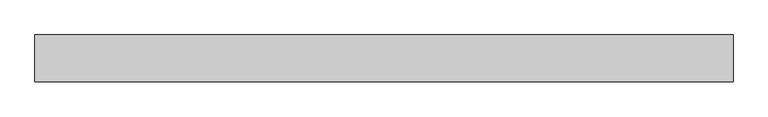
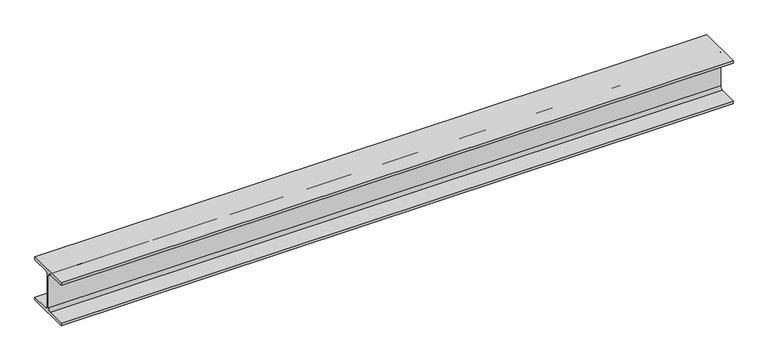
"""IFC4 building model written with IfcOpenShell, lengths in millimetres: beam geometry, 0912_Steel Framing_H-KSD3502 : H_SB_ASB_H-200x200x8x12."""

import ifcopenshell
import ifcopenshell.guid

model = None  # the IFC model being written
_history = None  # IfcOwnerHistory: only IFC2X3 demands one
_inside = {}  # id of a spatial element -> (the spatial element, [elements in it])
_under = {}  # id of a project, library or spatial element -> (it, [spatial elements below it])
_declared = {}  # id of a project -> (the project, [libraries it declares])
_typed = {}  # id of a type object -> (the type object, [elements of that type])
_made_of = {}  # id of a material, layer set ... -> (it, [elements and type objects made of it])


def new_model(schema):
    """Start an empty IFC model of exactly this schema.

    Asked for "IFC4X3", IfcOpenShell would pick the latest addendum, in which some entities
    have other attributes; the version numbers below select the first issue.
    IFC2X3 requires an IfcOwnerHistory on every rooted entity: one is made here for all.
    """
    global model, _history
    if schema == "IFC4X3":
        model = ifcopenshell.file(schema_version=(4, 3, 0, 0))
    else:
        model = ifcopenshell.file(schema=schema)
    _inside.clear()
    _under.clear()
    _declared.clear()
    _typed.clear()
    _made_of.clear()
    _history = None
    if model.schema == "IFC2X3":
        org = make("IfcOrganization", Name="unknown")
        user = make(
            "IfcPersonAndOrganization",
            ThePerson=make("IfcPerson", FamilyName="unknown"),
            TheOrganization=org,
        )
        app = make(
            "IfcApplication",
            ApplicationDeveloper=org,
            Version="unknown",
            ApplicationFullName="unknown",
            ApplicationIdentifier="unknown",
        )
        _history = make(
            "IfcOwnerHistory",
            OwningUser=user,
            OwningApplication=app,
            ChangeAction="ADDED",
            CreationDate=0,
        )
    return model


def make(cls, **values):
    """One entity of the class cls with the attributes given. An attribute that is None is left unset."""
    return model.create_entity(
        cls, **{name: value for name, value in values.items() if value is not None}
    )


def rooted(cls, **values):
    """An entity with a GlobalId (a new one), such as an element, a storey or a relation."""
    return make(cls, GlobalId=ifcopenshell.guid.new(), OwnerHistory=_history, **values)


def si_unit(unit_type, name, prefix=None):
    """IfcSIUnit, for example si_unit("LENGTHUNIT", "METRE", prefix="MILLI")."""
    return make("IfcSIUnit", UnitType=unit_type, Prefix=prefix, Name=name)


def assignment(units):
    """IfcUnitAssignment: the units of a project."""
    return None if units is None else make("IfcUnitAssignment", Units=units)


def point(xyz):
    """IfcCartesianPoint."""
    return None if xyz is None else make("IfcCartesianPoint", Coordinates=xyz)


def direction(xyz):
    """IfcDirection."""
    return None if xyz is None else make("IfcDirection", DirectionRatios=xyz)


def frame(location, z_axis=None, x_axis=None):
    """IfcAxis2Placement3D, a coordinate frame: its origin and axes. An axis left out is left unset."""
    return make(
        "IfcAxis2Placement3D",
        Location=point(location),
        Axis=direction(z_axis),
        RefDirection=direction(x_axis),
    )


def frame_2d(location, x_axis=None):
    """IfcAxis2Placement2D, a coordinate frame in the plane: its origin and x axis."""
    return make(
        "IfcAxis2Placement2D", Location=point(location), RefDirection=direction(x_axis)
    )


def origin():
    """The frame at (0, 0, 0) with its axes left unset."""
    return frame((0.0, 0.0, 0.0))


def place(relative_to, where):
    """IfcLocalPlacement: puts the frame where relative to a parent placement (None: the world)."""
    return make(
        "IfcLocalPlacement", PlacementRelTo=relative_to, RelativePlacement=where
    )


def context(
    kind, dimensions, precision=None, world=None, true_north=None, identifier=None
):
    """IfcGeometricRepresentationContext, for example the 3D "Model" context."""
    return make(
        "IfcGeometricRepresentationContext",
        ContextIdentifier=identifier,
        ContextType=kind,
        CoordinateSpaceDimension=dimensions,
        Precision=precision,
        WorldCoordinateSystem=world,
        TrueNorth=true_north,
    )


def project(units=None, contexts=None):
    """IfcProject with its units and contexts."""
    return rooted(
        "IfcProject",
        Name="project",
        RepresentationContexts=contexts,
        UnitsInContext=assignment(units),
    )


def spatial(cls, under=None, at=None, **own):
    """A site, building, storey or space (cls), placed at a placement, below another one or the project."""
    s = rooted(cls, ObjectPlacement=at, **own)
    if under is not None:
        _under.setdefault(under.id(), (under, []))[1].append(s)
    return s


def polyline(points):
    """IfcPolyline through the points."""
    return make("IfcPolyline", Points=[point(p) for p in points])


def circle_curve(where, radius):
    """IfcCircle in the frame where."""
    return make("IfcCircle", Position=where, Radius=radius)


def trimmed(basis, trim1, trim2, sense, master):
    """IfcTrimmedCurve: the piece of a basis curve between two trims."""
    return make(
        "IfcTrimmedCurve",
        BasisCurve=basis,
        Trim1=trim1,
        Trim2=trim2,
        SenseAgreement=sense,
        MasterRepresentation=master,
    )


def segment(curve, same_sense, transition):
    """IfcCompositeCurveSegment."""
    return make(
        "IfcCompositeCurveSegment",
        Transition=transition,
        SameSense=same_sense,
        ParentCurve=curve,
    )


def composite_curve(segments, self_intersect=None):
    """IfcCompositeCurve: segments joined end to end."""
    return make("IfcCompositeCurve", Segments=segments, SelfIntersect=self_intersect)


def outline(outer, holes=None, kind="AREA"):
    """IfcArbitraryClosedProfileDef: a profile drawn as a closed curve; with holes, ...WithVoids."""
    if holes is None:
        return make("IfcArbitraryClosedProfileDef", ProfileType=kind, OuterCurve=outer)
    return make(
        "IfcArbitraryProfileDefWithVoids",
        ProfileType=kind,
        OuterCurve=outer,
        InnerCurves=holes,
    )


def extrude(swept, where, along, depth):
    """IfcExtrudedAreaSolid: the profile swept, set in the frame where, extruded along a direction by depth."""
    return make(
        "IfcExtrudedAreaSolid",
        SweptArea=swept,
        Position=where,
        ExtrudedDirection=direction(along),
        Depth=depth,
    )


def shape(context_of_items, identifier, shape_type, items):
    """IfcShapeRepresentation: the items that make up one representation, for example the "Body"."""
    return make(
        "IfcShapeRepresentation",
        ContextOfItems=context_of_items,
        RepresentationIdentifier=identifier,
        RepresentationType=shape_type,
        Items=items,
    )


def source(mapping_origin, context_of_items, identifier, shape_type, items):
    """IfcRepresentationMap: a shape defined once, which mapped items show again and again."""
    return make(
        "IfcRepresentationMap",
        MappingOrigin=mapping_origin,
        MappedRepresentation=shape(context_of_items, identifier, shape_type, items),
    )


def transform(
    local_origin,
    x_axis=None,
    y_axis=None,
    z_axis=None,
    scale=None,
    scale2=None,
    scale3=None,
    uniform=True,
):
    """IfcCartesianTransformationOperator3D, or its non-uniform kind. x_axis, y_axis, z_axis: its Axis1, 2, 3."""
    if uniform:
        return make(
            "IfcCartesianTransformationOperator3D",
            Axis1=direction(x_axis),
            Axis2=direction(y_axis),
            LocalOrigin=point(local_origin),
            Scale=scale,
            Axis3=direction(z_axis),
        )
    return make(
        "IfcCartesianTransformationOperator3DnonUniform",
        Axis1=direction(x_axis),
        Axis2=direction(y_axis),
        LocalOrigin=point(local_origin),
        Scale=scale,
        Axis3=direction(z_axis),
        Scale2=scale2,
        Scale3=scale3,
    )


def mapped(mapping_source, mapping_target):
    """IfcMappedItem: shows the shape of a source again, moved by a transform."""
    return make(
        "IfcMappedItem", MappingSource=mapping_source, MappingTarget=mapping_target
    )


def made_of(thing, what):
    """Note that an element or type object is made of a material, layer set ...; save() writes the relation."""
    if what is not None:
        _made_of.setdefault(what.id(), (what, []))[1].append(thing)
    return thing


def element(
    cls,
    number,
    at=None,
    inside=None,
    cuts=None,
    type_object=None,
    material=None,
    context=None,
    identifier="Body",
    shape_type=None,
    held_by="IfcProductDefinitionShape",
    body=None,
    shapes=None,
    **own,
):
    """One element of the class cls, such as IfcWall. Its Tag is "e" and its number.

    at: its placement. inside: the storey or other place that contains it. cuts: it is an
    opening in that element (IfcRelVoidsElement). A single representation is given by context,
    identifier, shape_type and body (its items); several are given by shapes. held_by: the class
    of the entity that holds the representations. save() writes the other relations.
    """
    e = rooted(cls, Tag="e%d" % number, ObjectPlacement=at, **own)
    if body is not None:
        shapes = [shape(context, identifier, shape_type, body)]
    if shapes is not None:
        e.Representation = make(held_by, Representations=shapes)
    if inside is not None:
        _inside.setdefault(inside.id(), (inside, []))[1].append(e)
    if cuts is not None:
        rooted(
            "IfcRelVoidsElement", RelatingBuildingElement=cuts, RelatedOpeningElement=e
        )
    if type_object is not None:
        _typed.setdefault(type_object.id(), (type_object, []))[1].append(e)
    return made_of(e, material)


def aggregate(whole, parts):
    """IfcRelAggregates: a whole, such as a stair, and the parts it consists of."""
    return rooted("IfcRelAggregates", RelatingObject=whole, RelatedObjects=parts)


def save(model, path):
    """Write the relations noted so far, then the file.

    IfcRelAggregates (storeys below a building ...), IfcRelContainedInSpatialStructure (elements
    in a storey), IfcRelDefinesByType, IfcRelAssociatesMaterial and IfcRelDeclares: one each for
    every whole, place, type object, material and project.
    """
    for whole, parts in _under.values():
        aggregate(whole, parts)
    for where, things in _inside.values():
        rooted(
            "IfcRelContainedInSpatialStructure",
            RelatedElements=things,
            RelatingStructure=where,
        )
    for kind, things in _typed.values():
        rooted("IfcRelDefinesByType", RelatedObjects=things, RelatingType=kind)
    for what, things in _made_of.values():
        rooted("IfcRelAssociatesMaterial", RelatedObjects=things, RelatingMaterial=what)
    for by, libraries in _declared.values():
        rooted("IfcRelDeclares", RelatingContext=by, RelatedDefinitions=libraries)
    model.write(path)


def beam_a5566726(model_context):
    return source(origin(), model_context, "Body", "SweptSolid", [
        extrude(outline(composite_curve([segment(polyline([(100.0, -88.0), (100.0, -100.0), (-100.0, -100.0), (-100.0, -88.0), (-17.0, -88.0)]), True, "CONTINUOUS"), segment(trimmed(circle_curve(frame_2d((-17.0, -75.0)), 13.0), [point((-17.0, -88.0))], [point((-4.0, -75.0))], True, "CARTESIAN"), True, "CONTINUOUS"), segment(polyline([(-4.0, -75.0), (-4.0, 75.0)]), True, "CONTINUOUS"), segment(trimmed(circle_curve(frame_2d((-17.0, 75.0)), 13.0), [point((-4.0, 75.0))], [point((-17.0, 88.0))], True, "CARTESIAN"), True, "CONTINUOUS"), segment(polyline([(-17.0, 88.0), (-100.0, 88.0), (-100.0, 100.0), (100.0, 100.0), (100.0, 88.0), (17.0, 88.0)]), True, "CONTINUOUS"), segment(trimmed(circle_curve(frame_2d((17.0, 75.0)), 13.0), [point((17.0, 88.0))], [point((4.0, 75.0))], True, "CARTESIAN"), True, "CONTINUOUS"), segment(polyline([(4.0, 75.0), (4.0, -75.0)]), True, "CONTINUOUS"), segment(trimmed(circle_curve(frame_2d((17.0, -75.0)), 13.0), [point((4.0, -75.0))], [point((17.0, -88.0))], True, "CARTESIAN"), True, "CONTINUOUS"), segment(polyline([(17.0, -88.0), (100.0, -88.0)]), True, "CONTINUOUS")], self_intersect=False)), frame((-1443.5851857, 0.0, 0.0), z_axis=(1.0, 0.0, 0.0), x_axis=(0.0, 1.0, 0.0)), (0.0, 0.0, 1.0), 2972.6935261),
    ])


if __name__ == "__main__":
    model = new_model("IFC4")
    model_context = context("Model", 3, world=origin())
    ifc_project = project(units=[si_unit("LENGTHUNIT", "METRE", prefix="MILLI")], contexts=[model_context])
    site = spatial("IfcSite", under=ifc_project)
    building = spatial("IfcBuilding", under=site)
    placement = place(None, origin())
    beam_shape = beam_a5566726(model_context)
    element("IfcBeam", 1, ObjectType="0912_Steel Framing_H-KSD3502 : H_SB_ASB_H-200x200x8x12", at=placement, inside=building, context=model_context, shape_type="MappedRepresentation", body=[
        mapped(beam_shape, transform((0.0, 0.0, 0.0), x_axis=(1.0, 0.0, 0.0), y_axis=(0.0, 1.0, 0.0), z_axis=(0.0, 0.0, 1.0))),
    ])
    save(model, "model.ifc")

# Revit data of these elements
# Type "0912_Steel Framing_H-KSD3502 : H_SB_ASB_H-200x200x8x12"
#   H_WM Code_1 = "S01AA002-00001 | Main Steel Structure Fabrication Work | Shelter/Building | Medium Steel - Standard (90KG/M>Weight≥30KG/M) | Material: (   )"
#   H_WM Code_2 = "S03AA028-00001 | Main Steel Structure Erection Work | Shelter/Building | Medium Steel (90KG/M>Weight≥30KG/M) | Material: (   )"
#   H_WM Code_3 = "S01AA010-00001 | Main Steel Structure Fabrication Work | Shelter/Building | Steel Painting/Coating | for Non-Fireproofed Steel Surface, Surface Preparation, Primer, Second & Final Coat | Material: (   )"
#   H_Q'ty Cal Type Tag = "SB-Q2"
#   Width = 20.0 cm
#   Web Thickness = 0.8 cm
#   Web Fillet = 1.3 cm
#   Warping Constant = 141000.0 cm⁶
#   W = 0
#   Torsional Moment of Inertia = 26.2485 cm⁴
#   Section Area = 63.53 cm²
#   Plastic Modulus weak axis = 244.0 cm³
#   Plastic Modulus strong axis = 525.0 cm³
#   Perimeter = 1.16 m²/m
#   Nominal Weight = 49.90 kgf/m
#   Moment of Inertia weak axis = 1600.00 cm⁴
#   Moment of Inertia strong axis = 4720.00 cm⁴
#   Height = 20.0 cm
#   Flange Thickness = 1.2 cm
#   Elastic Modulus weak axis = 160.0 cm³
#   Elastic Modulus strong axis = 472.0 cm³
#   Centroid Vertical = 10.0 cm
#   Centroid Horizontal = 10.0 cm
#   Ix = 47200000
#   Length [instance default] = 1.5240 m
#   Zx = 525000
#   b = 0.2000 m
#   h = 0.2000 m
#   r = 0.0130 m
#   s = 0.0080 m
#   t = 0.0120 m
#   A = 0.006353 m²
#   Structural Material [instance default] = Steel, 45-345
#   Assembly Code = ""
# Element 1 (IfcBeam, "0912_Steel Framing_H-KSD3502 : H_SB_ASB_H-200x200x8x12")
#   Structural Material = none
# Materials
#   "Steel, 45-345": class "Metal", colour RGB 189 187 185, transparency 0, Description = "Steel 345 MPa", Cost = 0
